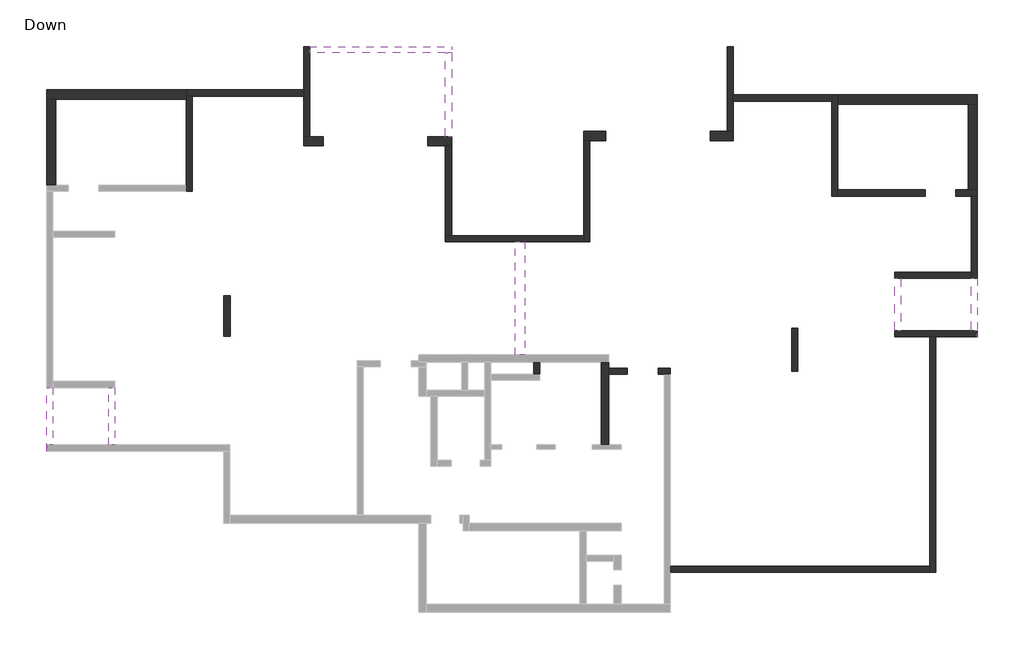
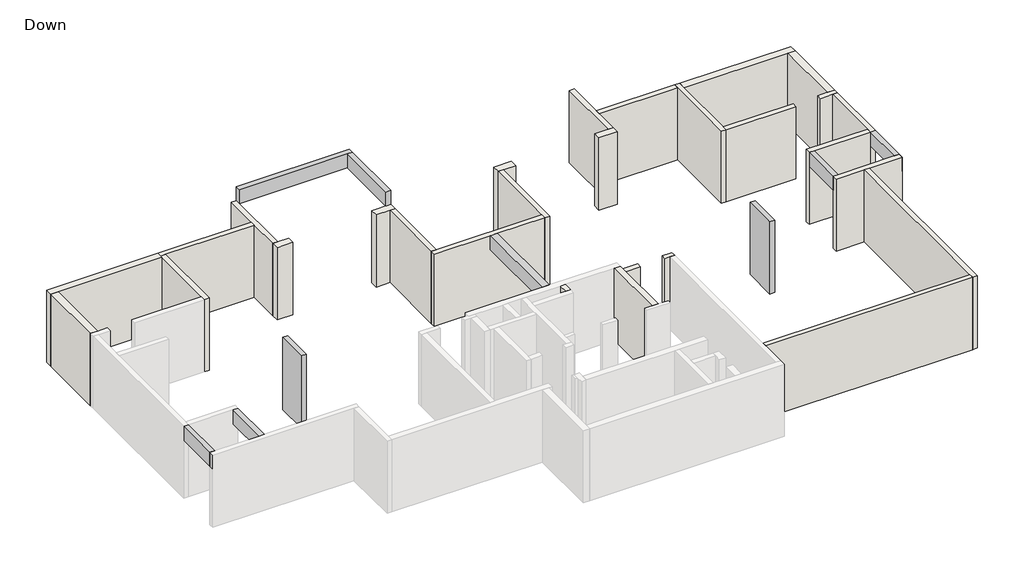
# One storey, part 2 of 2: 28 walls, 7 beams, 2 columns.
"""IFC4 building model written with IfcOpenShell, lengths in millimetres."""

from ifc_helpers import new_model, si_unit, frame, origin, origin_with_axes, place, context, project, spatial, polyline, outline, extrude, faceted_brep, element, save

model = new_model("IFC4")

# Units and contexts
model_context = context("Model", 3, world=origin())
ifc_project = project(units=[si_unit("LENGTHUNIT", "METRE", prefix="MILLI")], contexts=[model_context])

# Site, building, storey
site = spatial("IfcSite", under=ifc_project)
building = spatial("IfcBuilding", under=site)
storey = spatial("IfcBuildingStorey", under=building, Name="Down", Elevation=0.0)

# Beams
placement = place(None, origin())
element("IfcBeam", 1, ObjectType="Concrete Rectengular Beam : 20/60", at=placement, inside=storey, context=model_context, shape_type="Brep", body=[
    faceted_brep([(-15654.5633296, 19547.6197125, 3700.0), (-15654.5633296, 19547.6197125, 3100.0), (-15654.5633296, 19347.6197125, 3100.0), (-15654.5633296, 19347.6197125, 3700.0), (-11258.7738559, 19347.6197125, 3700.0), (-11058.7738559, 19347.6197125, 3700.0), (-11058.7738559, 19547.6197125, 3700.0), (-11258.7738559, 19347.6197125, 3100.0), (-11058.7738559, 19347.6197125, 3100.0), (-11058.7738559, 19547.6197125, 3100.0)], [[[0, 1, 2, 3]], [[0, 3, 4, 5, 6]], [[3, 2, 7, 8, 5, 4]], [[2, 1, 9, 8, 7]], [[1, 0, 6, 9]], [[6, 5, 8, 9]]]),
])
element("IfcBeam", 2, ObjectType="Concrete Rectengular Beam : 20/60", at=placement, inside=storey, context=model_context, shape_type="SweptSolid", body=[
    extrude(outline(polyline([(-11058.7738559, 16632.8828704), (-11258.7738559, 16632.8828704), (-11258.7738559, 19347.6197125), (-11058.7738559, 19347.6197125), (-11058.7738559, 16632.8828704)])), frame((0.0, 0.0, 3100.0), z_axis=(0.0, 0.0, 1.0), x_axis=(1.0, 0.0, 0.0)), (0.0, 0.0, 1.0), 600.0),
])
element("IfcBeam", 3, ObjectType="Concrete Rectengular Beam : 20/60", at=placement, inside=storey, context=model_context, shape_type="Brep", body=[
    faceted_brep([(3494.9103546, 12041.303923, 3100.0), (3294.9103546, 12041.303923, 3100.0), (3294.9103546, 10343.4091862, 3100.0), (3494.9103546, 10343.4091862, 3100.0), (3494.9103546, 12041.303923, 2500.0), (3494.9103546, 12041.303923, 2920.0), (3494.9103546, 10343.4091862, 2920.0), (3494.9103546, 10343.4091862, 2500.0), (3294.9103546, 12041.303923, 2500.0), (3294.9103546, 10343.4091862, 2500.0), (3294.9103546, 12041.303923, 2920.0), (3294.9103546, 10343.4091862, 2920.0)], [[[0, 1, 2, 3]], [[4, 5, 0, 3, 6, 7]], [[8, 4, 7, 9]], [[2, 1, 10, 8, 9, 11]], [[1, 0, 5, 4, 8, 10]], [[3, 2, 11, 9, 7, 6]]]),
])
element("IfcBeam", 4, ObjectType="Concrete Rectengular Beam : 20/60", at=placement, inside=storey, context=model_context, shape_type="Brep", body=[
    faceted_brep([(5979.1208809, 10143.4091862, 3100.0), (5981.2261441, 10143.4091862, 3100.0), (5981.2261441, 12041.303923, 3100.0), (5782.2787756, 12041.303923, 3100.0), (5781.2261441, 12041.303923, 3100.0), (5781.2261441, 10343.4091862, 3100.0), (5979.1208809, 10343.4091862, 3100.0), (5981.2261441, 10143.4091862, 2500.0), (5981.2261441, 12041.303923, 2500.0), (5979.1208809, 10143.4091862, 2500.0), (5979.1208809, 10343.4091862, 2500.0), (5781.2261441, 10343.4091862, 2500.0), (5781.2261441, 12041.303923, 2500.0), (5781.2261441, 10343.4091862, 2920.0), (5781.2261441, 12041.303923, 2920.0)], [[[0, 1, 2, 3, 4, 5, 6]], [[1, 7, 8, 2]], [[7, 9, 10, 11, 12, 8]], [[11, 13, 5, 4, 14, 12]], [[7, 1, 0, 9]], [[10, 6, 5, 13, 11]], [[6, 10, 9, 0]], [[2, 8, 12, 14, 4, 3]]]),
])
element("IfcBeam", 5, ObjectType="Concrete Rectengular Beam : 20/60", at=placement, inside=storey, context=model_context, shape_type="Brep", body=[
    faceted_brep([(-21970.3528033, 8497.0933967, 3100.0), (-22170.3528033, 8497.0933967, 3100.0), (-22170.3528033, 6638.1460283, 3100.0), (-21970.3528033, 6638.1460283, 3100.0), (-22170.3528033, 8497.0933967, 2920.0), (-22170.3528033, 8497.0933967, 2500.0), (-22170.3528033, 6638.1460283, 2500.0), (-22170.3528033, 6638.1460283, 2920.0), (-21970.3528033, 8497.0933967, 2500.0), (-21970.3528033, 6638.1460283, 2500.0), (-21970.3528033, 6638.1460283, 2920.0), (-21970.3528033, 8497.0933967, 2920.0)], [[[0, 1, 2, 3]], [[1, 4, 5, 6, 7, 2]], [[5, 8, 9, 6]], [[0, 3, 10, 9, 8, 11]], [[1, 0, 11, 8, 5, 4]], [[3, 2, 7, 6, 9, 10]]]),
])
element("IfcBeam", 6, ObjectType="Concrete Rectengular Beam : 20/60", at=placement, inside=storey, context=model_context, shape_type="Brep", body=[
    faceted_brep([(-24180.8791191, 6438.1460283, 3100.0), (-24178.7738559, 6438.1460283, 3100.0), (-24178.7738559, 6638.1460283, 3100.0), (-23980.8791191, 6638.1460283, 3100.0), (-23980.8791191, 8497.0933967, 3100.0), (-24180.8791191, 8497.0933967, 3100.0), (-24180.8791191, 6438.1460283, 2500.0), (-24180.8791191, 8497.0933967, 2500.0), (-24178.7738559, 6438.1460283, 2500.0), (-23980.8791191, 8497.0933967, 2500.0), (-23980.8791191, 6638.1460283, 2500.0), (-24178.7738559, 6638.1460283, 2500.0), (-23980.8791191, 6638.1460283, 2920.0), (-23980.8791191, 8497.0933967, 2920.0)], [[[0, 1, 2, 3, 4, 5]], [[6, 0, 5, 7]], [[8, 6, 7, 9, 10, 11]], [[3, 12, 10, 9, 13, 4]], [[0, 6, 8, 1]], [[2, 11, 10, 12, 3]], [[11, 2, 1, 8]], [[5, 4, 13, 9, 7]]]),
])
element("IfcBeam", 7, ObjectType="Concrete Rectengular Beam : 30/60", at=placement, inside=storey, context=model_context, shape_type="Brep", body=[
    faceted_brep([(-8691.4054349, 13221.303923, 3100.0), (-8991.4054349, 13221.303923, 3100.0), (-8991.4054349, 9562.3565546, 3100.0), (-8691.4054349, 9562.3565546, 3100.0), (-8691.4054349, 13221.303923, 2500.0), (-8691.4054349, 13221.303923, 2920.0), (-8691.4054349, 9562.3565546, 2920.0), (-8691.4054349, 9562.3565546, 2500.0), (-8991.4054349, 13221.303923, 2500.0), (-8991.4054349, 9562.3565546, 2500.0), (-8991.4054349, 13221.303923, 2920.0), (-8991.4054349, 9562.3565546, 2920.0)], [[[0, 1, 2, 3]], [[4, 5, 0, 3, 6, 7]], [[8, 4, 7, 9]], [[1, 10, 8, 9, 11, 2]], [[1, 0, 5, 4, 8, 10]], [[3, 2, 11, 9, 7, 6]]]),
])

# Columns
element("IfcColumn", 8, ObjectType="Concrete Rectengular Column : 20/130", at=placement, inside=storey, context=model_context, shape_type="Brep", body=[
    faceted_brep([(-18235.4928274, 11466.5670809, 0.0), (-18235.4928274, 10166.5670809, 0.0), (-18435.4928274, 10166.5670809, 0.0), (-18435.4928274, 11466.5670809, 0.0), (-18235.4928274, 11466.5670809, 3100.0), (-18235.4928274, 10166.5670809, 3100.0), (-18235.4928274, 10166.5670809, 2920.0), (-18235.4928274, 11466.5670809, 2920.0), (-18435.4928274, 10166.5670809, 3100.0), (-18435.4928274, 10166.5670809, 2920.0), (-18435.4928274, 11466.5670809, 3100.0), (-18435.4928274, 11466.5670809, 2920.0)], [[[0, 1, 2, 3]], [[4, 5, 6, 1, 0, 7]], [[5, 8, 9, 2, 1, 6]], [[8, 10, 11, 3, 2, 9]], [[10, 4, 7, 0, 3, 11]], [[4, 10, 8, 5]]]),
])
element("IfcColumn", 9, ObjectType="Concrete Rectengular Column : 20/140", at=placement, inside=storey, context=model_context, shape_type="Brep", body=[
    faceted_brep([(162.2787756, 10426.8302388, 0.0), (162.2787756, 9026.8302388, 0.0), (-37.7212244, 9026.8302388, 0.0), (-37.7212244, 10426.8302388, 0.0), (162.2787756, 10426.8302388, 3100.0), (162.2787756, 9026.8302388, 3100.0), (162.2787756, 9026.8302388, 2920.0), (162.2787756, 10426.8302388, 2920.0), (-37.7212244, 9026.8302388, 3100.0), (-37.7212244, 9026.8302388, 2920.0), (-37.7212244, 10426.8302388, 3100.0), (-37.7212244, 10426.8302388, 2920.0)], [[[0, 1, 2, 3]], [[4, 5, 6, 1, 0, 7]], [[5, 8, 9, 2, 1, 6]], [[8, 10, 11, 3, 2, 9]], [[10, 4, 7, 0, 3, 11]], [[4, 10, 8, 5]]]),
])

# Walls
element("IfcWall", 10, ObjectType="20", at=placement, inside=storey, context=model_context, shape_type="Brep", body=[
    faceted_brep([(-15854.5633296, 18143.4091862, 0.0), (-19660.8791191, 18143.4091862, 0.0), (-19660.8791191, 18143.4091862, 3100.0), (-15854.5633296, 18143.4091862, 3100.0), (-15854.5633296, 17943.4091862, 0.0), (-15854.5633296, 17943.4091862, 2920.0), (-15854.5633296, 17943.4091862, 3100.0), (-19460.8791191, 17943.4091862, 3100.0), (-19660.8791191, 17943.4091862, 3100.0), (-19660.8791191, 17943.4091862, 0.0), (-19460.8791191, 17943.4091862, 0.0)], [[[0, 1, 2, 3]], [[4, 5, 6, 7, 8, 9, 10]], [[1, 0, 4, 10, 9]], [[3, 2, 8, 7, 6]], [[2, 1, 9, 8]], [[0, 3, 6, 5, 4]]]),
])
element("IfcWall", 11, ObjectType="20", at=placement, inside=storey, context=model_context, shape_type="Brep", body=[
    faceted_brep([(-19660.8791191, 17943.4091862, 0.0), (-19660.8791191, 17843.4091862, 0.0), (-19660.8791191, 15061.303923, 0.0), (-19660.8791191, 14861.303923, 0.0), (-19660.8791191, 14861.303923, 3100.0), (-19660.8791191, 15061.303923, 3100.0), (-19660.8791191, 17843.4091862, 3100.0), (-19660.8791191, 17943.4091862, 3100.0), (-19460.8791191, 17943.4091862, 0.0), (-19460.8791191, 17943.4091862, 2920.0), (-19460.8791191, 17943.4091862, 3100.0), (-19460.8791191, 14861.303923, 3100.0), (-19460.8791191, 14861.303923, 2920.0), (-19460.8791191, 14861.303923, 0.0)], [[[0, 1, 2, 3, 4, 5, 6, 7]], [[8, 9, 10, 11, 12, 13]], [[3, 2, 1, 0, 8, 13]], [[7, 6, 5, 4, 11, 10]], [[0, 7, 10, 9, 8]], [[4, 3, 13, 12, 11]]]),
])
element("IfcWall", 12, ObjectType="20", at=placement, inside=storey, context=model_context, shape_type="Brep", body=[
    faceted_brep([(-15654.5633296, 16632.8828704, 0.0), (-15654.5633296, 19545.5144494, 0.0), (-15654.5633296, 19545.5144494, 3100.0), (-15654.5633296, 16632.8828704, 3100.0), (-15654.5633296, 16632.8828704, 2920.0), (-15854.5633296, 16632.8828704, 0.0), (-15854.5633296, 16632.8828704, 3100.0), (-15854.5633296, 17943.4091862, 3100.0), (-15854.5633296, 18143.4091862, 3100.0), (-15854.5633296, 19545.5144494, 3100.0), (-15854.5633296, 19545.5144494, 0.0), (-15854.5633296, 18143.4091862, 0.0), (-15854.5633296, 17943.4091862, 0.0)], [[[0, 1, 2, 3, 4]], [[5, 6, 7, 8, 9, 10, 11, 12]], [[1, 0, 5, 12, 11, 10]], [[2, 1, 10, 9]], [[3, 2, 9, 8, 7, 6]], [[0, 4, 3, 6, 5]]]),
])
element("IfcWall", 13, ObjectType="20", at=placement, inside=storey, context=model_context, shape_type="Brep", body=[
    faceted_brep([(-11258.7738559, 16332.8828704, 0.0), (-11258.7738559, 13421.303923, 0.0), (-11258.7738559, 13421.303923, 3100.0), (-11258.7738559, 16332.8828704, 3100.0), (-11258.7738559, 16332.8828704, 2920.0), (-11058.7738559, 16332.8828704, 0.0), (-11058.7738559, 16332.8828704, 3100.0), (-11058.7738559, 13421.303923, 3100.0), (-11058.7738559, 13421.303923, 0.0)], [[[0, 1, 2, 3, 4]], [[5, 6, 7, 8]], [[1, 0, 5, 8]], [[3, 2, 7, 6]], [[0, 4, 3, 6, 5]], [[2, 1, 8, 7]]]),
])
element("IfcWall", 14, ObjectType="20", at=placement, inside=storey, context=model_context, shape_type="Brep", body=[
    faceted_brep([(-11258.7738559, 13221.303923, 0.0), (-6772.4580665, 13221.303923, 0.0), (-6772.4580665, 13221.303923, 3100.0), (-8691.4054349, 13221.303923, 3100.0), (-8991.4054349, 13221.303923, 3100.0), (-11258.7738559, 13221.303923, 3100.0), (-11258.7738559, 13221.303923, 2920.0), (-11258.7738559, 13421.303923, 0.0), (-11258.7738559, 13421.303923, 3100.0), (-11058.7738559, 13421.303923, 3100.0), (-6772.4580665, 13421.303923, 3100.0), (-6772.4580665, 13421.303923, 0.0), (-11058.7738559, 13421.303923, 0.0)], [[[0, 1, 2, 3, 4, 5, 6]], [[7, 8, 9, 10, 11, 12]], [[1, 0, 7, 12, 11]], [[5, 4, 3, 2, 10, 9, 8]], [[0, 6, 5, 8, 7]], [[2, 1, 11, 10]]]),
])
element("IfcWall", 15, ObjectType="20", at=placement, inside=storey, context=model_context, shape_type="Brep", body=[
    faceted_brep([(1262.2787756, 17983.4091862, 0.0), (1262.2787756, 17783.4091862, 0.0), (1262.2787756, 14701.303923, 0.0), (1262.2787756, 14701.303923, 2920.0), (1262.2787756, 14701.303923, 3100.0), (1262.2787756, 17783.4091862, 3100.0), (1262.2787756, 17983.4091862, 3100.0), (1462.2787756, 17983.4091862, 0.0), (1462.2787756, 17983.4091862, 3100.0), (1462.2787756, 17683.4091862, 3100.0), (1462.2787756, 14901.303923, 3100.0), (1462.2787756, 14701.303923, 3100.0), (1462.2787756, 14701.303923, 0.0), (1462.2787756, 14901.303923, 0.0), (1462.2787756, 17683.4091862, 0.0)], [[[0, 1, 2, 3, 4, 5, 6]], [[7, 8, 9, 10, 11, 12, 13, 14]], [[2, 1, 0, 7, 14, 13, 12]], [[6, 5, 4, 11, 10, 9, 8]], [[0, 6, 8, 7]], [[4, 3, 2, 12, 11]]]),
])
element("IfcWall", 16, ObjectType="20", at=placement, inside=storey, context=model_context, shape_type="Brep", body=[
    faceted_brep([(1462.2787756, 14701.303923, 0.0), (4292.2787756, 14701.303923, 0.0), (4292.2787756, 14701.303923, 2920.0), (4292.2787756, 14701.303923, 3100.0), (1462.2787756, 14701.303923, 3100.0), (1462.2787756, 14901.303923, 0.0), (1462.2787756, 14901.303923, 2920.0), (1462.2787756, 14901.303923, 3100.0), (4292.2787756, 14901.303923, 3100.0), (4292.2787756, 14901.303923, 2920.0), (4292.2787756, 14901.303923, 0.0)], [[[0, 1, 2, 3, 4]], [[5, 6, 7, 8, 9, 10]], [[1, 0, 5, 10]], [[3, 2, 1, 10, 9, 8]], [[4, 3, 8, 7]], [[0, 4, 7, 6, 5]]]),
])
element("IfcWall", 17, ObjectType="20", at=placement, inside=storey, context=model_context, shape_type="Brep", body=[
    faceted_brep([(5285.4366704, 14701.303923, 0.0), (5782.2787756, 14701.303923, 0.0), (5982.2787756, 14701.303923, 0.0), (5982.2787756, 14701.303923, 3100.0), (5782.2787756, 14701.303923, 3100.0), (5285.4366704, 14701.303923, 3100.0), (5285.4366704, 14701.303923, 2920.0), (5285.4366704, 14901.303923, 0.0), (5285.4366704, 14901.303923, 2920.0), (5285.4366704, 14901.303923, 3100.0), (5680.1735125, 14901.303923, 3100.0), (5980.1735125, 14901.303923, 3100.0), (5982.2787756, 14901.303923, 3100.0), (5982.2787756, 14901.303923, 0.0), (5980.1735125, 14901.303923, 0.0), (5680.1735125, 14901.303923, 0.0)], [[[0, 1, 2, 3, 4, 5, 6]], [[7, 8, 9, 10, 11, 12, 13, 14, 15]], [[2, 1, 0, 7, 15, 14, 13]], [[5, 4, 3, 12, 11, 10, 9]], [[0, 6, 5, 9, 8, 7]], [[3, 2, 13, 12]]]),
])
element("IfcWall", 18, ObjectType="20", at=placement, inside=storey, context=model_context, shape_type="Brep", body=[
    faceted_brep([(5782.2787756, 14701.303923, 0.0), (5782.2787756, 12241.303923, 0.0), (5782.2787756, 12041.303923, 0.0), (5782.2787756, 12041.303923, 3100.0), (5782.2787756, 12241.303923, 3100.0), (5782.2787756, 14701.303923, 3100.0), (5782.2787756, 14701.303923, 2920.0), (5982.2787756, 14701.303923, 0.0), (5982.2787756, 14701.303923, 3100.0), (5982.2787756, 12041.303923, 3100.0), (5982.2787756, 12041.303923, 0.0), (5981.2261441, 12041.303923, 3100.0)], [[[0, 1, 2, 3, 4, 5, 6]], [[7, 8, 9, 10]], [[2, 1, 0, 7, 10]], [[5, 4, 3, 11, 9, 8]], [[0, 6, 5, 8, 7]], [[3, 2, 10, 9, 11]]]),
])
element("IfcWall", 19, ObjectType="20", at=placement, inside=storey, context=model_context, shape_type="Brep", body=[
    faceted_brep([(1262.2787756, 17983.4091862, 0.0), (-1922.7212244, 17983.4091862, 0.0), (-1922.7212244, 17983.4091862, 3100.0), (1262.2787756, 17983.4091862, 3100.0), (1262.2787756, 17783.4091862, 0.0), (1262.2787756, 17783.4091862, 2920.0), (1262.2787756, 17783.4091862, 3100.0), (-1922.7212244, 17783.4091862, 3100.0), (-1922.7212244, 17783.4091862, 2920.0), (-1922.7212244, 17783.4091862, 0.0)], [[[0, 1, 2, 3]], [[4, 5, 6, 7, 8, 9]], [[1, 0, 4, 9]], [[3, 2, 7, 6]], [[2, 1, 9, 8, 7]], [[0, 3, 6, 5, 4]]]),
])
element("IfcWall", 20, ObjectType="20", at=placement, inside=storey, context=model_context, shape_type="Brep", body=[
    faceted_brep([(-1922.7212244, 16800.2512915, 0.0), (-1922.7212244, 17783.4091862, 0.0), (-1922.7212244, 17983.4091862, 0.0), (-1922.7212244, 19545.5144494, 0.0), (-1922.7212244, 19545.5144494, 3100.0), (-1922.7212244, 17983.4091862, 3100.0), (-1922.7212244, 17783.4091862, 3100.0), (-1922.7212244, 16800.2512915, 3100.0), (-2122.7212244, 16800.2512915, 0.0), (-2122.7212244, 16800.2512915, 2920.0), (-2122.7212244, 16800.2512915, 3100.0), (-2122.7212244, 19545.5144494, 3100.0), (-2122.7212244, 19545.5144494, 0.0)], [[[0, 1, 2, 3, 4, 5, 6, 7]], [[8, 9, 10, 11, 12]], [[3, 2, 1, 0, 8, 12]], [[4, 3, 12, 11]], [[7, 6, 5, 4, 11, 10]], [[0, 7, 10, 9, 8]]]),
])
element("IfcWall", 21, ObjectType="20", at=placement, inside=storey, context=model_context, shape_type="Brep", body=[
    faceted_brep([(-6772.4580665, 16500.2512915, 0.0), (-6772.4580665, 13421.303923, 0.0), (-6772.4580665, 13221.303923, 0.0), (-6772.4580665, 13221.303923, 3100.0), (-6772.4580665, 13421.303923, 3100.0), (-6772.4580665, 16500.2512915, 3100.0), (-6572.4580665, 16500.2512915, 0.0), (-6572.4580665, 16500.2512915, 2920.0), (-6572.4580665, 16500.2512915, 3100.0), (-6572.4580665, 13221.303923, 3100.0), (-6572.4580665, 13221.303923, 2920.0), (-6572.4580665, 13221.303923, 0.0)], [[[0, 1, 2, 3, 4, 5]], [[6, 7, 8, 9, 10, 11]], [[2, 1, 0, 6, 11]], [[5, 4, 3, 9, 8]], [[0, 5, 8, 7, 6]], [[3, 2, 11, 10, 9]]]),
])
element("IfcWall", 22, ObjectType="20", at=placement, inside=storey, context=model_context, shape_type="Brep", body=[
    faceted_brep([(5782.2787756, 12241.303923, 0.0), (3294.9103546, 12241.303923, 0.0), (3294.9103546, 12241.303923, 2920.0), (3294.9103546, 12241.303923, 3100.0), (5782.2787756, 12241.303923, 3100.0), (5782.2787756, 12241.303923, 2920.0), (5782.2787756, 12041.303923, 0.0), (5782.2787756, 12041.303923, 3100.0), (5781.2261441, 12041.303923, 3100.0), (3494.9103546, 12041.303923, 3100.0), (3294.9103546, 12041.303923, 3100.0), (3294.9103546, 12041.303923, 0.0)], [[[0, 1, 2, 3, 4, 5]], [[6, 7, 8, 9, 10, 11]], [[1, 0, 6, 11]], [[3, 2, 1, 11, 10]], [[4, 3, 10, 9, 8, 7]], [[0, 5, 4, 7, 6]]]),
])
element("IfcWall", 23, ObjectType="20", at=placement, inside=storey, context=model_context, shape_type="Brep", body=[
    faceted_brep([(3294.9103546, 10143.4091862, 0.0), (4435.9629862, 10143.4091862, 0.0), (4635.9629862, 10143.4091862, 0.0), (5979.1208809, 10143.4091862, 0.0), (5979.1208809, 10143.4091862, 3100.0), (4635.9629862, 10143.4091862, 3100.0), (4435.9629862, 10143.4091862, 3100.0), (3294.9103546, 10143.4091862, 3100.0), (3294.9103546, 10143.4091862, 2920.0), (3294.9103546, 10343.4091862, 0.0), (3294.9103546, 10343.4091862, 3100.0), (3494.9103546, 10343.4091862, 3100.0), (5781.2261441, 10343.4091862, 3100.0), (5979.1208809, 10343.4091862, 3100.0), (5979.1208809, 10343.4091862, 0.0)], [[[0, 1, 2, 3, 4, 5, 6, 7, 8]], [[9, 10, 11, 12, 13, 14]], [[3, 2, 1, 0, 9, 14]], [[4, 3, 14, 13]], [[7, 6, 5, 4, 13, 12, 11, 10]], [[0, 8, 7, 10, 9]]]),
])
element("IfcWall", 24, ObjectType="20", at=placement, inside=storey, context=model_context, shape_type="Brep", body=[
    faceted_brep([(4435.9629862, 10143.4091862, 0.0), (4435.9629862, 2716.0407652, 0.0), (4435.9629862, 2516.0407652, 0.0), (4435.9629862, 2516.0407652, 3100.0), (4435.9629862, 2716.0407652, 3100.0), (4435.9629862, 10143.4091862, 3100.0), (4435.9629862, 10143.4091862, 2920.0), (4635.9629862, 10143.4091862, 0.0), (4635.9629862, 10143.4091862, 3100.0), (4635.9629862, 2516.0407652, 3100.0), (4635.9629862, 2516.0407652, 0.0)], [[[0, 1, 2, 3, 4, 5, 6]], [[7, 8, 9, 10]], [[2, 1, 0, 7, 10]], [[5, 4, 3, 9, 8]], [[0, 6, 5, 8, 7]], [[3, 2, 10, 9]]]),
])
element("IfcWall", 25, ObjectType="20", at=placement, inside=storey, context=model_context, shape_type="Brep", body=[
    faceted_brep([(4435.9629862, 2716.0407652, 0.0), (-3966.142277, 2716.0407652, 0.0), (-3966.142277, 2716.0407652, 2920.0), (-3966.142277, 2716.0407652, 3100.0), (4435.9629862, 2716.0407652, 3100.0), (4435.9629862, 2716.0407652, 2920.0), (4435.9629862, 2516.0407652, 0.0), (4435.9629862, 2516.0407652, 3100.0), (-3966.142277, 2516.0407652, 3100.0), (-3966.142277, 2516.0407652, 0.0)], [[[0, 1, 2, 3, 4, 5]], [[6, 7, 8, 9]], [[1, 0, 6, 9]], [[4, 3, 8, 7]], [[0, 5, 4, 7, 6]], [[3, 2, 1, 9, 8]]]),
])
element("IfcWall", 26, ObjectType="20", at=placement, inside=storey, context=model_context, shape_type="Brep", body=[
    faceted_brep([(-3966.142277, 9130.7776073, 0.0), (-4366.142277, 9130.7776073, 0.0), (-4366.142277, 9130.7776073, 2920.0), (-4366.142277, 9130.7776073, 3100.0), (-3966.142277, 9130.7776073, 3100.0), (-3966.142277, 9130.7776073, 2920.0), (-3966.142277, 8930.7776073, 0.0), (-3966.142277, 8930.7776073, 3100.0), (-4166.142277, 8930.7776073, 3100.0), (-4366.142277, 8930.7776073, 3100.0), (-4366.142277, 8930.7776073, 2920.0), (-4366.142277, 8930.7776073, 0.0), (-4166.142277, 8930.7776073, 0.0)], [[[0, 1, 2, 3, 4, 5]], [[6, 7, 8, 9, 10, 11, 12]], [[1, 0, 6, 12, 11]], [[3, 2, 1, 11, 10, 9]], [[4, 3, 9, 8, 7]], [[0, 5, 4, 7, 6]]]),
])
element("IfcWall", 27, ObjectType="20", at=placement, inside=storey, context=model_context, shape_type="Brep", body=[
    faceted_brep([(-5359.8264875, 9130.7776073, 0.0), (-5957.7212244, 9130.7776073, 0.0), (-5957.7212244, 9130.7776073, 2920.0), (-5957.7212244, 9130.7776073, 3100.0), (-5359.8264875, 9130.7776073, 3100.0), (-5359.8264875, 9130.7776073, 2920.0), (-5359.8264875, 8930.7776073, 0.0), (-5359.8264875, 8930.7776073, 2920.0), (-5359.8264875, 8930.7776073, 3100.0), (-5957.7212244, 8930.7776073, 3100.0), (-5957.7212244, 8930.7776073, 2920.0), (-5957.7212244, 8930.7776073, 0.0)], [[[0, 1, 2, 3, 4, 5]], [[6, 7, 8, 9, 10, 11]], [[1, 0, 6, 11]], [[4, 3, 9, 8]], [[0, 5, 4, 8, 7, 6]], [[3, 2, 1, 11, 10, 9]]]),
])
element("IfcWall", 28, ObjectType="20", at=placement, inside=storey, context=model_context, shape_type="SweptSolid", body=[
    extrude(outline(polyline([(-8195.6159612, 9312.3565546), (-8195.6159612, 8932.8828704), (-8395.6159612, 8932.8828704), (-8395.6159612, 9312.3565546), (-8195.6159612, 9312.3565546)])), origin_with_axes(), (0.0, 0.0, 1.0), 3100.0),
])
element("IfcWall", 29, ObjectType="25", at=placement, inside=storey, context=model_context, shape_type="Brep", body=[
    faceted_brep([(-6207.7212244, 9312.3565546, 0.0), (-6207.7212244, 6644.9881336, 0.0), (-6207.7212244, 6644.9881336, 3100.0), (-6207.7212244, 9312.3565546, 3100.0), (-5957.7212244, 9312.3565546, 0.0), (-5957.7212244, 9312.3565546, 3100.0), (-5957.7212244, 9130.7776073, 3100.0), (-5957.7212244, 8930.7776073, 3100.0), (-5957.7212244, 6644.9881336, 3100.0), (-5957.7212244, 6644.9881336, 2920.0), (-5957.7212244, 6644.9881336, 0.0), (-5957.7212244, 8930.7776073, 0.0), (-5957.7212244, 9130.7776073, 0.0)], [[[0, 1, 2, 3]], [[4, 5, 6, 7, 8, 9, 10, 11, 12]], [[1, 0, 4, 12, 11, 10]], [[3, 2, 8, 7, 6, 5]], [[2, 1, 10, 9, 8]], [[0, 3, 5, 4]]]),
])
element("IfcWall", 30, ObjectType="30", at=placement, inside=storey, context=model_context, shape_type="Brep", body=[
    faceted_brep([(-19660.8791191, 18143.4091862, 0.0), (-24178.7738559, 18143.4091862, 0.0), (-24178.7738559, 18143.4091862, 3100.0), (-19660.8791191, 18143.4091862, 3100.0), (-19660.8791191, 17843.4091862, 0.0), (-19660.8791191, 17843.4091862, 2920.0), (-19660.8791191, 17843.4091862, 3100.0), (-23878.7738559, 17843.4091862, 3100.0), (-24178.7738559, 17843.4091862, 3100.0), (-24178.7738559, 17843.4091862, 0.0), (-23878.7738559, 17843.4091862, 0.0), (-19660.8791191, 17943.4091862, 0.0), (-19660.8791191, 17943.4091862, 3100.0)], [[[0, 1, 2, 3]], [[4, 5, 6, 7, 8, 9, 10]], [[1, 0, 11, 4, 10, 9]], [[3, 2, 8, 7, 6, 12]], [[0, 3, 12, 6, 5, 4, 11]], [[2, 1, 9, 8]]]),
])
element("IfcWall", 31, ObjectType="30", at=placement, inside=storey, context=model_context, shape_type="Brep", body=[
    faceted_brep([(-24178.7738559, 17843.4091862, 0.0), (-24178.7738559, 15061.303923, 0.0), (-24178.7738559, 15061.303923, 3100.0), (-24178.7738559, 17843.4091862, 3100.0), (-23878.7738559, 17843.4091862, 0.0), (-23878.7738559, 17843.4091862, 2920.0), (-23878.7738559, 17843.4091862, 3100.0), (-23878.7738559, 15061.303923, 3100.0), (-23878.7738559, 15061.303923, 2920.0), (-23878.7738559, 15061.303923, 0.0)], [[[0, 1, 2, 3]], [[4, 5, 6, 7, 8, 9]], [[1, 0, 4, 9]], [[3, 2, 7, 6]], [[0, 3, 6, 5, 4]], [[2, 1, 9, 8, 7]]]),
])
element("IfcWall", 32, ObjectType="30", at=placement, inside=storey, context=model_context, shape_type="Brep", body=[
    faceted_brep([(-15854.5633296, 16332.8828704, 0.0), (-15208.2475402, 16332.8828704, 0.0), (-15208.2475402, 16332.8828704, 2920.0), (-15208.2475402, 16332.8828704, 3100.0), (-15854.5633296, 16332.8828704, 3100.0), (-15854.5633296, 16332.8828704, 2920.0), (-15854.5633296, 16632.8828704, 0.0), (-15854.5633296, 16632.8828704, 3100.0), (-15654.5633296, 16632.8828704, 3100.0), (-15208.2475402, 16632.8828704, 3100.0), (-15208.2475402, 16632.8828704, 2920.0), (-15208.2475402, 16632.8828704, 0.0), (-15654.5633296, 16632.8828704, 0.0)], [[[0, 1, 2, 3, 4, 5]], [[6, 7, 8, 9, 10, 11, 12]], [[1, 0, 6, 12, 11]], [[3, 2, 1, 11, 10, 9]], [[4, 3, 9, 8, 7]], [[0, 5, 4, 7, 6]]]),
])
element("IfcWall", 33, ObjectType="30", at=placement, inside=storey, context=model_context, shape_type="Brep", body=[
    faceted_brep([(-11825.0896454, 16332.8828704, 0.0), (-11258.7738559, 16332.8828704, 0.0), (-11058.7738559, 16332.8828704, 0.0), (-11058.7738559, 16332.8828704, 3100.0), (-11258.7738559, 16332.8828704, 3100.0), (-11825.0896454, 16332.8828704, 3100.0), (-11825.0896454, 16332.8828704, 2920.0), (-11825.0896454, 16632.8828704, 0.0), (-11825.0896454, 16632.8828704, 2920.0), (-11825.0896454, 16632.8828704, 3100.0), (-11058.7738559, 16632.8828704, 3100.0), (-11058.7738559, 16632.8828704, 2920.0), (-11058.7738559, 16632.8828704, 0.0)], [[[0, 1, 2, 3, 4, 5, 6]], [[7, 8, 9, 10, 11, 12]], [[2, 1, 0, 7, 12]], [[5, 4, 3, 10, 9]], [[0, 6, 5, 9, 8, 7]], [[3, 2, 12, 11, 10]]]),
])
element("IfcWall", 34, ObjectType="30", at=placement, inside=storey, context=model_context, shape_type="Brep", body=[
    faceted_brep([(1462.2787756, 17683.4091862, 0.0), (5680.1735125, 17683.4091862, 0.0), (5980.1735125, 17683.4091862, 0.0), (5980.1735125, 17683.4091862, 3100.0), (5680.1735125, 17683.4091862, 3100.0), (1462.2787756, 17683.4091862, 3100.0), (1462.2787756, 17683.4091862, 2920.0), (1462.2787756, 17983.4091862, 0.0), (1462.2787756, 17983.4091862, 3100.0), (5980.1735125, 17983.4091862, 3100.0), (5980.1735125, 17983.4091862, 0.0)], [[[0, 1, 2, 3, 4, 5, 6]], [[7, 8, 9, 10]], [[2, 1, 0, 7, 10]], [[5, 4, 3, 9, 8]], [[0, 6, 5, 8, 7]], [[3, 2, 10, 9]]]),
])
element("IfcWall", 35, ObjectType="30", at=placement, inside=storey, context=model_context, shape_type="Brep", body=[
    faceted_brep([(5680.1735125, 17683.4091862, 0.0), (5680.1735125, 14901.303923, 0.0), (5680.1735125, 14901.303923, 2920.0), (5680.1735125, 14901.303923, 3100.0), (5680.1735125, 17683.4091862, 3100.0), (5680.1735125, 17683.4091862, 2920.0), (5980.1735125, 17683.4091862, 0.0), (5980.1735125, 17683.4091862, 3100.0), (5980.1735125, 14901.303923, 3100.0), (5980.1735125, 14901.303923, 0.0)], [[[0, 1, 2, 3, 4, 5]], [[6, 7, 8, 9]], [[1, 0, 6, 9]], [[4, 3, 8, 7]], [[0, 5, 4, 7, 6]], [[3, 2, 1, 9, 8]]]),
])
element("IfcWall", 36, ObjectType="30", at=placement, inside=storey, context=model_context, shape_type="Brep", body=[
    faceted_brep([(-1922.7212244, 16800.2512915, 0.0), (-2122.7212244, 16800.2512915, 0.0), (-2672.7212244, 16800.2512915, 0.0), (-2672.7212244, 16800.2512915, 2920.0), (-2672.7212244, 16800.2512915, 3100.0), (-2122.7212244, 16800.2512915, 3100.0), (-1922.7212244, 16800.2512915, 3100.0), (-1922.7212244, 16500.2512915, 0.0), (-1922.7212244, 16500.2512915, 2920.0), (-1922.7212244, 16500.2512915, 3100.0), (-2672.7212244, 16500.2512915, 3100.0), (-2672.7212244, 16500.2512915, 2920.0), (-2672.7212244, 16500.2512915, 0.0)], [[[0, 1, 2, 3, 4, 5, 6]], [[7, 8, 9, 10, 11, 12]], [[2, 1, 0, 7, 12]], [[4, 3, 2, 12, 11, 10]], [[6, 5, 4, 10, 9]], [[0, 6, 9, 8, 7]]]),
])
element("IfcWall", 37, ObjectType="30", at=placement, inside=storey, context=model_context, shape_type="Brep", body=[
    faceted_brep([(-6057.4580665, 16800.2512915, 0.0), (-6772.4580665, 16800.2512915, 0.0), (-6772.4580665, 16800.2512915, 2920.0), (-6772.4580665, 16800.2512915, 3100.0), (-6057.4580665, 16800.2512915, 3100.0), (-6057.4580665, 16800.2512915, 2920.0), (-6057.4580665, 16500.2512915, 0.0), (-6057.4580665, 16500.2512915, 2920.0), (-6057.4580665, 16500.2512915, 3100.0), (-6572.4580665, 16500.2512915, 3100.0), (-6772.4580665, 16500.2512915, 3100.0), (-6772.4580665, 16500.2512915, 0.0), (-6572.4580665, 16500.2512915, 0.0)], [[[0, 1, 2, 3, 4, 5]], [[6, 7, 8, 9, 10, 11, 12]], [[1, 0, 6, 12, 11]], [[4, 3, 10, 9, 8]], [[0, 5, 4, 8, 7, 6]], [[3, 2, 1, 11, 10]]]),
])

save(model, "model.ifc")

# Revit data of these elements
# Type "Concrete Rectengular Beam : 20/60"
#   Length [instance default] = 152.4 cm
#   b = 20 cm
#   h = 60 cm
#   Structural Material [instance default] = Concrete
#   Assembly Code = ""
# Type "Concrete Rectengular Beam : 30/60"
#   Length [instance default] = 152.4 cm
#   b = 30 cm
#   h = 60 cm
#   Structural Material [instance default] = Concrete
#   Assembly Code = ""
# Type "Concrete Rectengular Column : 20/130"
#   b = 20 cm
#   h = 130 cm
#   Structural Material [instance default] = Concrete
# Type "Concrete Rectengular Column : 20/140"
#   b = 20 cm
#   h = 140 cm
#   Structural Material [instance default] = Concrete
# Type "20"
#   Layers, outside or top first: 20 cm "Concrete" (function 1)
# Type "25"
#   Layers, outside or top first: 25 cm "Concrete" (function 1)
# Type "30"
#   Layers, outside or top first: 30 cm "Concrete" (function 1)
# Element 1 (IfcBeam, "Concrete Rectengular Beam : 20/60")
#   Comments = ""
#   Mark = "B1"
#   SOFiSTiK_AMG_Comments = ""
#   SOFiSTiK_AMG_Scheduled = yes
#   SOFiSTiK_AMG_Adjusted = yes
#   Structural Material = Concrete
#   Phase Created = New Construction
#   Materials on its faces: "Concrete"
# Element 2 (IfcBeam, "Concrete Rectengular Beam : 20/60")
#   Comments = ""
#   Mark = "B2"
#   SOFiSTiK_AMG_Comments = ""
#   SOFiSTiK_AMG_Scheduled = yes
#   SOFiSTiK_AMG_Adjusted = yes
#   Structural Material = Concrete
#   Phase Created = New Construction
#   Materials on its faces: "Concrete"
# Element 3 (IfcBeam, "Concrete Rectengular Beam : 20/60")
#   Comments = ""
#   Mark = "B5"
#   SOFiSTiK_AMG_Comments = ""
#   SOFiSTiK_AMG_Scheduled = yes
#   SOFiSTiK_AMG_Adjusted = yes
#   Structural Material = Concrete
#   Phase Created = New Construction
#   Materials on its faces: "Concrete"
# Element 4 (IfcBeam, "Concrete Rectengular Beam : 20/60")
#   Comments = ""
#   Mark = "B6"
#   SOFiSTiK_AMG_Comments = ""
#   SOFiSTiK_AMG_Scheduled = yes
#   SOFiSTiK_AMG_Adjusted = yes
#   Structural Material = Concrete
#   Phase Created = New Construction
#   Materials on its faces: "Concrete"
# Element 5 (IfcBeam, "Concrete Rectengular Beam : 20/60")
#   Comments = ""
#   Mark = "B7"
#   SOFiSTiK_AMG_Comments = ""
#   SOFiSTiK_AMG_Scheduled = yes
#   SOFiSTiK_AMG_Adjusted = yes
#   Structural Material = Concrete
#   Phase Created = New Construction
#   Materials on its faces: "Concrete"
# Element 6 (IfcBeam, "Concrete Rectengular Beam : 20/60")
#   Comments = ""
#   Mark = "B8"
#   SOFiSTiK_AMG_Comments = ""
#   SOFiSTiK_AMG_Scheduled = yes
#   SOFiSTiK_AMG_Adjusted = yes
#   Structural Material = Concrete
#   Phase Created = New Construction
#   Materials on its faces: "Concrete"
# Element 7 (IfcBeam, "Concrete Rectengular Beam : 30/60")
#   Comments = ""
#   Mark = "B9"
#   SOFiSTiK_AMG_Comments = ""
#   SOFiSTiK_AMG_Scheduled = yes
#   SOFiSTiK_AMG_Adjusted = yes
#   Structural Material = Concrete
#   Phase Created = New Construction
#   Materials on its faces: "Concrete"
# Element 8 (IfcColumn, "Concrete Rectengular Column : 20/130")
#   Comments = ""
#   Mark = "C1"
#   SOFiSTiK_AMG_Comments = ""
#   SOFiSTiK_AMG_Scheduled = yes
#   SOFiSTiK_AMG_Adjusted = yes
#   Structural Material = Concrete
#   Phase Created = New Construction
#   Materials on its faces: "Concrete"
# Element 9 (IfcColumn, "Concrete Rectengular Column : 20/140")
#   Comments = ""
#   Mark = "C2"
#   SOFiSTiK_AMG_Comments = ""
#   SOFiSTiK_AMG_Scheduled = yes
#   SOFiSTiK_AMG_Adjusted = yes
#   Structural Material = Concrete
#   Phase Created = New Construction
#   Materials on its faces: "Concrete"
# Element 10 (IfcWall, "20")
#   Comments = ""
#   Mark = "W1"
#   SOFiSTiK_EdgeZones = "W1"
#   SOFiSTiK_AMG_Comments = ""
#   Top Offset = 0 cm
#   Base Offset = 0 cm
#   wall height = 310 cm
#   SOFiSTiK_AMG_Scheduled = yes
#   SOFiSTiK_AMG_Adjusted = yes
#   Phase Created = New Construction
#   Base Constraint = Down
#   Top Constraint = Typical Floor
#   Materials on its faces: "Concrete"
# Element 11 (IfcWall, "20")
#   Comments = ""
#   Mark = "W2"
#   SOFiSTiK_EdgeZones = "W2"
#   SOFiSTiK_AMG_Comments = ""
#   Top Offset = 0 cm
#   Base Offset = 0 cm
#   wall height = 310 cm
#   SOFiSTiK_AMG_Scheduled = yes
#   SOFiSTiK_AMG_Adjusted = yes
#   Phase Created = New Construction
#   Base Constraint = Down
#   Top Constraint = Typical Floor
#   Materials on its faces: "Concrete"
# Element 12 (IfcWall, "20")
#   Comments = ""
#   Mark = "W14"
#   SOFiSTiK_EdgeZones = "W16"
#   SOFiSTiK_AMG_Comments = ""
#   Top Offset = 0 cm
#   Base Offset = 0 cm
#   wall height = 310 cm
#   SOFiSTiK_AMG_Scheduled = yes
#   SOFiSTiK_AMG_Adjusted = yes
#   Phase Created = New Construction
#   Base Constraint = Down
#   Top Constraint = Typical Floor
#   Materials on its faces: "Concrete"
# Element 13 (IfcWall, "20")
#   Comments = ""
#   Mark = "W15"
#   SOFiSTiK_EdgeZones = "W17"
#   SOFiSTiK_AMG_Comments = ""
#   Top Offset = 0 cm
#   Base Offset = 0 cm
#   wall height = 310 cm
#   SOFiSTiK_AMG_Scheduled = yes
#   SOFiSTiK_AMG_Adjusted = yes
#   Phase Created = New Construction
#   Base Constraint = Down
#   Top Constraint = Typical Floor
#   Materials on its faces: "Concrete"
# Element 14 (IfcWall, "20")
#   Comments = ""
#   Mark = "W16"
#   SOFiSTiK_EdgeZones = "W18"
#   SOFiSTiK_AMG_Comments = ""
#   Top Offset = 0 cm
#   Base Offset = 0 cm
#   wall height = 310 cm
#   SOFiSTiK_AMG_Scheduled = yes
#   SOFiSTiK_AMG_Adjusted = yes
#   Phase Created = New Construction
#   Base Constraint = Down
#   Top Constraint = Typical Floor
#   Materials on its faces: "Concrete"
# Element 15 (IfcWall, "20")
#   Comments = ""
#   Mark = "W17"
#   SOFiSTiK_EdgeZones = "W20"
#   SOFiSTiK_AMG_Comments = ""
#   Top Offset = 0 cm
#   Base Offset = 0 cm
#   wall height = 310 cm
#   SOFiSTiK_AMG_Scheduled = yes
#   SOFiSTiK_AMG_Adjusted = yes
#   Phase Created = New Construction
#   Base Constraint = Down
#   Top Constraint = Typical Floor
#   Materials on its faces: "Concrete"
# Element 16 (IfcWall, "20")
#   Comments = ""
#   Mark = "W18"
#   SOFiSTiK_EdgeZones = "W21"
#   SOFiSTiK_AMG_Comments = ""
#   Top Offset = 0 cm
#   Base Offset = 0 cm
#   wall height = 310 cm
#   SOFiSTiK_AMG_Scheduled = yes
#   SOFiSTiK_AMG_Adjusted = yes
#   Phase Created = New Construction
#   Base Constraint = Down
#   Top Constraint = Typical Floor
#   Materials on its faces: "Concrete"
# Element 17 (IfcWall, "20")
#   Comments = ""
#   Mark = "W19"
#   SOFiSTiK_EdgeZones = "W22"
#   SOFiSTiK_AMG_Comments = ""
#   Top Offset = 0 cm
#   Base Offset = 0 cm
#   wall height = 310 cm
#   SOFiSTiK_AMG_Scheduled = yes
#   SOFiSTiK_AMG_Adjusted = yes
#   Phase Created = New Construction
#   Base Constraint = Down
#   Top Constraint = Typical Floor
#   Materials on its faces: "Concrete"
# Element 18 (IfcWall, "20")
#   Comments = ""
#   Mark = "W20"
#   SOFiSTiK_EdgeZones = "W23"
#   SOFiSTiK_AMG_Comments = ""
#   Top Offset = 0 cm
#   Base Offset = 0 cm
#   wall height = 310 cm
#   SOFiSTiK_AMG_Scheduled = yes
#   SOFiSTiK_AMG_Adjusted = yes
#   Phase Created = New Construction
#   Base Constraint = Down
#   Top Constraint = Typical Floor
#   Materials on its faces: "Concrete"
# Element 19 (IfcWall, "20")
#   Comments = ""
#   Mark = "W21"
#   SOFiSTiK_EdgeZones = "W24"
#   SOFiSTiK_AMG_Comments = ""
#   Top Offset = 0 cm
#   Base Offset = 0 cm
#   wall height = 310 cm
#   SOFiSTiK_AMG_Scheduled = yes
#   SOFiSTiK_AMG_Adjusted = yes
#   Phase Created = New Construction
#   Base Constraint = Down
#   Top Constraint = Typical Floor
#   Materials on its faces: "Concrete"
# Element 20 (IfcWall, "20")
#   Comments = ""
#   Mark = "W22"
#   SOFiSTiK_EdgeZones = "W26"
#   SOFiSTiK_AMG_Comments = ""
#   Top Offset = 0 cm
#   Base Offset = 0 cm
#   wall height = 310 cm
#   SOFiSTiK_AMG_Scheduled = yes
#   SOFiSTiK_AMG_Adjusted = yes
#   Phase Created = New Construction
#   Base Constraint = Down
#   Top Constraint = Typical Floor
#   Materials on its faces: "Concrete"
# Element 21 (IfcWall, "20")
#   Comments = ""
#   Mark = "W23"
#   SOFiSTiK_EdgeZones = "W27"
#   SOFiSTiK_AMG_Comments = ""
#   Top Offset = 0 cm
#   Base Offset = 0 cm
#   wall height = 310 cm
#   SOFiSTiK_AMG_Scheduled = yes
#   SOFiSTiK_AMG_Adjusted = yes
#   Phase Created = New Construction
#   Base Constraint = Down
#   Top Constraint = Typical Floor
#   Materials on its faces: "Concrete"
# Element 22 (IfcWall, "20")
#   Comments = ""
#   Mark = "W25"
#   SOFiSTiK_EdgeZones = "W29"
#   SOFiSTiK_AMG_Comments = ""
#   Top Offset = 0 cm
#   Base Offset = 0 cm
#   wall height = 310 cm
#   SOFiSTiK_AMG_Scheduled = yes
#   SOFiSTiK_AMG_Adjusted = yes
#   Phase Created = New Construction
#   Base Constraint = Down
#   Top Constraint = Typical Floor
#   Materials on its faces: "Concrete"
# Element 23 (IfcWall, "20")
#   Comments = ""
#   Mark = "W26"
#   SOFiSTiK_EdgeZones = "W30"
#   SOFiSTiK_AMG_Comments = ""
#   Top Offset = 0 cm
#   Base Offset = 0 cm
#   wall height = 310 cm
#   SOFiSTiK_AMG_Scheduled = yes
#   SOFiSTiK_AMG_Adjusted = yes
#   Phase Created = New Construction
#   Base Constraint = Down
#   Top Constraint = Typical Floor
#   Materials on its faces: "Concrete"
# Element 24 (IfcWall, "20")
#   Comments = ""
#   Mark = "W27"
#   SOFiSTiK_EdgeZones = "W31"
#   SOFiSTiK_AMG_Comments = ""
#   Top Offset = 0 cm
#   Base Offset = 0 cm
#   wall height = 310 cm
#   SOFiSTiK_AMG_Scheduled = yes
#   SOFiSTiK_AMG_Adjusted = yes
#   Phase Created = New Construction
#   Base Constraint = Down
#   Top Constraint = Typical Floor
#   Materials on its faces: "Concrete"
# Element 25 (IfcWall, "20")
#   Comments = ""
#   Mark = "W28"
#   SOFiSTiK_EdgeZones = "W32"
#   SOFiSTiK_AMG_Comments = ""
#   Top Offset = 0 cm
#   Base Offset = 0 cm
#   wall height = 310 cm
#   SOFiSTiK_AMG_Scheduled = yes
#   SOFiSTiK_AMG_Adjusted = yes
#   Phase Created = New Construction
#   Base Constraint = Down
#   Top Constraint = Typical Floor
#   Materials on its faces: "Concrete"
# Element 26 (IfcWall, "20")
#   Comments = ""
#   Mark = "W30"
#   SOFiSTiK_EdgeZones = "W35"
#   SOFiSTiK_AMG_Comments = ""
#   Top Offset = 0 cm
#   Base Offset = 0 cm
#   wall height = 310 cm
#   SOFiSTiK_AMG_Scheduled = yes
#   SOFiSTiK_AMG_Adjusted = yes
#   Phase Created = New Construction
#   Base Constraint = Down
#   Top Constraint = Typical Floor
#   Materials on its faces: "Concrete"
# Element 27 (IfcWall, "20")
#   Comments = ""
#   Mark = "W31"
#   SOFiSTiK_EdgeZones = "W36"
#   SOFiSTiK_AMG_Comments = ""
#   Top Offset = 0 cm
#   Base Offset = 0 cm
#   wall height = 310 cm
#   SOFiSTiK_AMG_Scheduled = yes
#   SOFiSTiK_AMG_Adjusted = yes
#   Phase Created = New Construction
#   Base Constraint = Down
#   Top Constraint = Typical Floor
#   Materials on its faces: "Concrete"
# Element 28 (IfcWall, "20")
#   Comments = ""
#   Mark = "W35"
#   SOFiSTiK_EdgeZones = "W40"
#   SOFiSTiK_AMG_Comments = ""
#   Top Offset = 0 cm
#   Base Offset = 0 cm
#   wall height = 310 cm
#   SOFiSTiK_AMG_Scheduled = yes
#   SOFiSTiK_AMG_Adjusted = yes
#   Phase Created = New Construction
#   Base Constraint = Down
#   Top Constraint = Typical Floor
#   Materials on its faces: "Concrete"
# Element 29 (IfcWall, "25")
#   Comments = ""
#   Mark = "W50"
#   SOFiSTiK_EdgeZones = "W57"
#   SOFiSTiK_AMG_Comments = ""
#   Top Offset = 0 cm
#   Base Offset = 0 cm
#   wall height = 310 cm
#   SOFiSTiK_AMG_Scheduled = yes
#   SOFiSTiK_AMG_Adjusted = yes
#   Phase Created = New Construction
#   Base Constraint = Down
#   Top Constraint = Typical Floor
#   Materials on its faces: "Concrete"
# Element 30 (IfcWall, "30")
#   Comments = ""
#   Mark = "W53"
#   SOFiSTiK_EdgeZones = "W60"
#   SOFiSTiK_AMG_Comments = ""
#   Top Offset = 0 cm
#   Base Offset = 0 cm
#   wall height = 310 cm
#   SOFiSTiK_AMG_Scheduled = yes
#   SOFiSTiK_AMG_Adjusted = yes
#   Phase Created = New Construction
#   Base Constraint = Down
#   Top Constraint = Typical Floor
#   Materials on its faces: "Concrete"
# Element 31 (IfcWall, "30")
#   Comments = ""
#   Mark = "W54"
#   SOFiSTiK_EdgeZones = "W61"
#   SOFiSTiK_AMG_Comments = ""
#   Top Offset = 0 cm
#   Base Offset = 0 cm
#   wall height = 310 cm
#   SOFiSTiK_AMG_Scheduled = yes
#   SOFiSTiK_AMG_Adjusted = yes
#   Phase Created = New Construction
#   Base Constraint = Down
#   Top Constraint = Typical Floor
#   Materials on its faces: "Concrete"
# Element 32 (IfcWall, "30")
#   Comments = ""
#   Mark = "W55"
#   SOFiSTiK_EdgeZones = "W62"
#   SOFiSTiK_AMG_Comments = ""
#   Top Offset = 0 cm
#   Base Offset = 0 cm
#   wall height = 310 cm
#   SOFiSTiK_AMG_Scheduled = yes
#   SOFiSTiK_AMG_Adjusted = yes
#   Phase Created = New Construction
#   Base Constraint = Down
#   Top Constraint = Typical Floor
#   Materials on its faces: "Concrete"
# Element 33 (IfcWall, "30")
#   Comments = ""
#   Mark = "W56"
#   SOFiSTiK_EdgeZones = "W63"
#   SOFiSTiK_AMG_Comments = ""
#   Top Offset = 0 cm
#   Base Offset = 0 cm
#   wall height = 310 cm
#   SOFiSTiK_AMG_Scheduled = yes
#   SOFiSTiK_AMG_Adjusted = yes
#   Phase Created = New Construction
#   Base Constraint = Down
#   Top Constraint = Typical Floor
#   Materials on its faces: "Concrete"
# Element 34 (IfcWall, "30")
#   Comments = ""
#   Mark = "W57"
#   SOFiSTiK_EdgeZones = "W64"
#   SOFiSTiK_AMG_Comments = ""
#   Top Offset = 0 cm
#   Base Offset = 0 cm
#   wall height = 310 cm
#   SOFiSTiK_AMG_Scheduled = yes
#   SOFiSTiK_AMG_Adjusted = yes
#   Phase Created = New Construction
#   Base Constraint = Down
#   Top Constraint = Typical Floor
#   Materials on its faces: "Concrete"
# Element 35 (IfcWall, "30")
#   Comments = ""
#   Mark = "W58"
#   SOFiSTiK_EdgeZones = "W65"
#   SOFiSTiK_AMG_Comments = ""
#   Top Offset = 0 cm
#   Base Offset = 0 cm
#   wall height = 310 cm
#   SOFiSTiK_AMG_Scheduled = yes
#   SOFiSTiK_AMG_Adjusted = yes
#   Phase Created = New Construction
#   Base Constraint = Down
#   Top Constraint = Typical Floor
#   Materials on its faces: "Concrete"
# Element 36 (IfcWall, "30")
#   Comments = ""
#   Mark = "W59"
#   SOFiSTiK_EdgeZones = "W66"
#   SOFiSTiK_AMG_Comments = ""
#   Top Offset = 0 cm
#   Base Offset = 0 cm
#   wall height = 310 cm
#   SOFiSTiK_AMG_Scheduled = yes
#   SOFiSTiK_AMG_Adjusted = yes
#   Phase Created = New Construction
#   Base Constraint = Down
#   Top Constraint = Typical Floor
#   Materials on its faces: "Concrete"
# Element 37 (IfcWall, "30")
#   Comments = ""
#   Mark = "W60"
#   SOFiSTiK_EdgeZones = "W67"
#   SOFiSTiK_AMG_Comments = ""
#   Top Offset = 0 cm
#   Base Offset = 0 cm
#   wall height = 310 cm
#   SOFiSTiK_AMG_Scheduled = yes
#   SOFiSTiK_AMG_Adjusted = yes
#   Phase Created = New Construction
#   Base Constraint = Down
#   Top Constraint = Typical Floor
#   Materials on its faces: "Concrete"
# Materials
#   "Concrete": class "Concrete", colour RGB 192 192 192, transparency 0, Keynote = "01000", Description = "Cast-in-place concrete", Cost = 0
